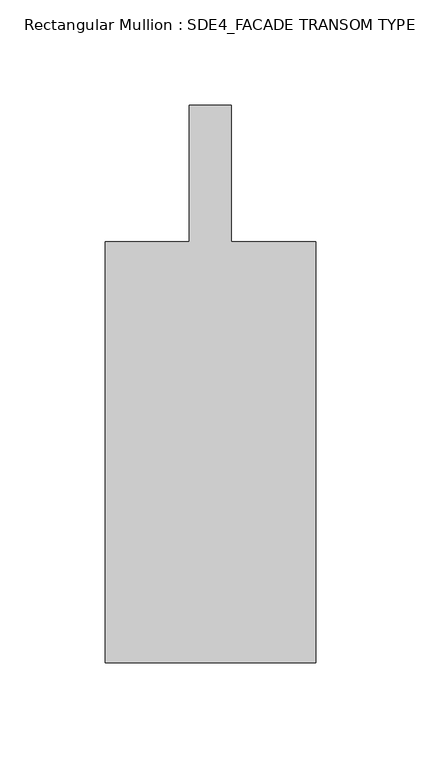
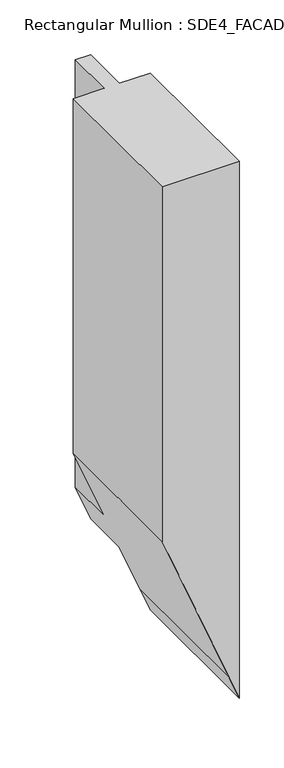
"""IFC4 building model written with IfcOpenShell, lengths in millimetres: member geometry, Rectangular Mullion : SDE4_FACADE TRANSOM TYPE 2."""

from ifc_helpers import new_model, si_unit, origin, place, context, project, spatial, faceted_brep, source, transform, mapped, element, save


def rectangular_mullion_sde4_facade_transom_type_2_08ee4245(model_context):
    return source(origin(), model_context, "Body", "Brep", [
        faceted_brep([(50.0, -132.5, 0.0), (50.0, 67.5, 0.0), (10.0, 67.5, 0.0), (10.0, 132.5, 0.0), (-10.0, 132.5, 0.0), (-10.0, 67.5, 0.0), (-50.0, 67.5, 0.0), (-50.0, -132.5, 0.0), (50.0, -132.5, -737.2330639), (50.0, 67.5, -737.2330639), (37.1390676, 67.5, -705.080733), (10.0, 67.5, -637.2330639), (10.0, 132.5, -637.2330639), (-10.0, 132.5, -587.2330639), (-10.0, 67.5, -587.2330639), (-50.0, 67.5, -487.2330639), (-50.0, -132.5, -487.2330639), (37.1390676, -132.5, -705.080733)], [[[0, 1, 2, 3, 4, 5, 6, 7]], [[1, 0, 8, 9]], [[2, 1, 9, 10, 11]], [[3, 2, 11, 12]], [[4, 3, 12, 13]], [[5, 4, 13, 14]], [[6, 5, 14, 15]], [[7, 6, 15, 16]], [[0, 7, 16, 17, 8]], [[8, 17, 10, 9]], [[17, 16, 15, 14, 13, 12, 11, 10]]]),
    ])


if __name__ == "__main__":
    model = new_model("IFC4")
    model_context = context("Model", 3, world=origin())
    ifc_project = project(units=[si_unit("LENGTHUNIT", "METRE", prefix="MILLI")], contexts=[model_context])
    site = spatial("IfcSite", under=ifc_project)
    building = spatial("IfcBuilding", under=site)
    placement = place(None, origin())
    rectangular_mullion_sde4_facade_transom_type_2_shape = rectangular_mullion_sde4_facade_transom_type_2_08ee4245(model_context)
    element("IfcMember", 1, ObjectType="Rectangular Mullion : SDE4_FACADE TRANSOM TYPE 2", at=placement, inside=building, context=model_context, shape_type="MappedRepresentation", body=[
        mapped(rectangular_mullion_sde4_facade_transom_type_2_shape, transform((0.0, 0.0, 0.0), x_axis=(1.0, 0.0, 0.0), y_axis=(0.0, 1.0, 0.0), z_axis=(0.0, 0.0, 1.0))),
    ])
    save(model, "model.ifc")

# Revit data of these elements
# Type "Rectangular Mullion : SDE4_FACADE TRANSOM TYPE 2"
#   built-in parameter 1007322 = 0.869423 (stored number, unit not read)
#   built-in parameter 1007321 = 0.164042 (stored number, unit not read)
#   built-in parameter 1007320 = 0.164042 (stored number, unit not read)
